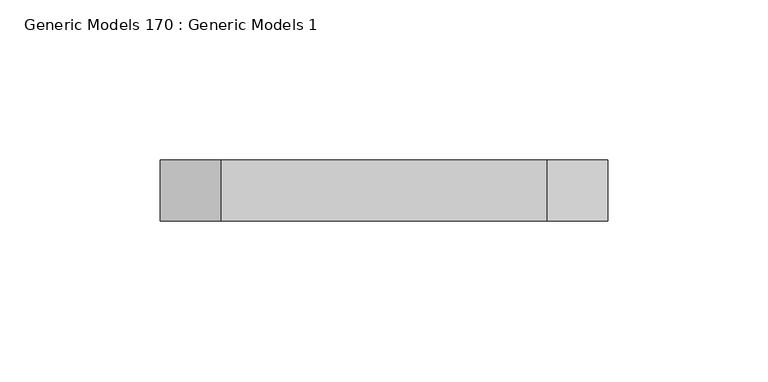
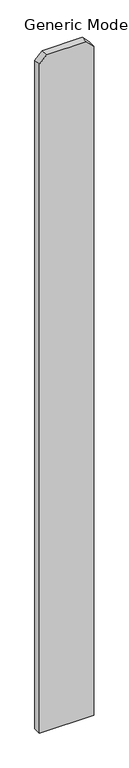
"""IFC4 building model written with IfcOpenShell, lengths in millimetres: proxy geometry, Generic Models 170 : Generic Models 1."""

from ifc_helpers import new_model, si_unit, frame, origin, place, context, project, spatial, polyline, outline, extrude, source, transform, mapped, element, save


def generic_models_170_generic_models_1_1b954c43(model_context):
    return source(origin(), model_context, "Body", "SweptSolid", [
        extrude(outline(polyline([(76.2, 55903.8125), (1885.95, 55903.8125), (1905.0, 55884.7625), (1905.0, 55783.1625), (1885.95, 55764.1125), (76.2, 55764.1125), (76.2, 55903.8125)])), frame((0.0, 547.6875, 0.0), z_axis=(0.0, 1.0, 0.0), x_axis=(0.0, 0.0, 1.0)), (0.0, 0.0, 1.0), 19.05),
    ])


if __name__ == "__main__":
    model = new_model("IFC4")
    model_context = context("Model", 3, world=origin())
    ifc_project = project(units=[si_unit("LENGTHUNIT", "METRE", prefix="MILLI")], contexts=[model_context])
    site = spatial("IfcSite", under=ifc_project)
    building = spatial("IfcBuilding", under=site)
    placement = place(None, origin())
    generic_models_170_generic_models_1_shape = generic_models_170_generic_models_1_1b954c43(model_context)
    element("IfcBuildingElementProxy", 1, Name="Generic Models 170 : Generic Models 1", ObjectType="Generic Models 170 : Generic Models 1", at=placement, inside=building, context=model_context, shape_type="MappedRepresentation", body=[
        mapped(generic_models_170_generic_models_1_shape, transform((0.0, 0.0, 0.0), x_axis=(1.0, 0.0, 0.0), y_axis=(0.0, 1.0, 0.0), z_axis=(0.0, 0.0, 1.0))),
    ])
    save(model, "model.ifc")

# Revit data of these elements
# Element 1 (IfcBuildingElementProxy, "Generic Models 170 : Generic Models 1")
#   Materials on its faces: "VERTICAL 1X6 CEDAR PLANKS W/ CLEAR WOOD SEALER"
# Materials
#   "VERTICAL 1X6 CEDAR PLANKS W/ CLEAR WOOD SEALER": class "Wood", colour RGB 234 198 147, transparency 0, Description = "Pinus Echinata", Cost = 0
